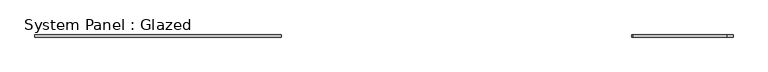
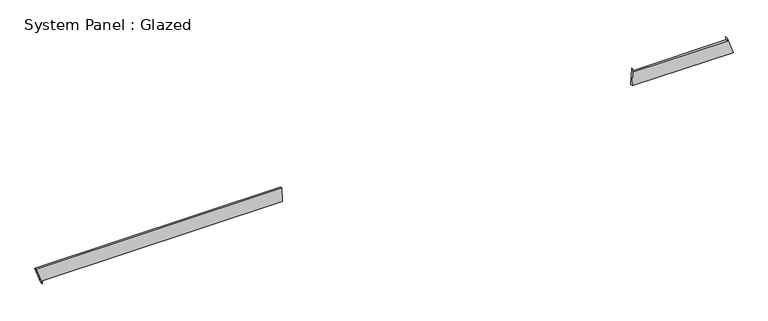
"""IFC4 building model written with IfcOpenShell, lengths in millimetres: plate geometry, System Panel : Glazed."""

from ifc_helpers import new_model, si_unit, frame, origin, place, context, project, spatial, polyline, outline, extrude, source, transform, mapped, element, save


def system_panel_glazed_9f0471fb(model_context):
    return source(origin(), model_context, "Body", "SweptSolid", [
        extrude(outline(polyline([(35.3553391, 2859.8495797), (35.3553391, 4027.1832678), (235.4605257, 3957.794267), (200.1051866, 3957.7948933), (200.0858758, 2867.7205954), (235.4412148, 2867.7199691), (35.3553391, 2859.8495797)])), frame((0.0, -49.5, 0.0), z_axis=(0.0, 1.0, 0.0), x_axis=(0.0, 0.0, 1.0)), (0.0, 0.0, 1.0), 25.0),
        extrude(outline(polyline([(0.0, -3957.4553629), (35.3553391, -3957.4553629), (35.3553391, -1184.8268191), (200.0140372, -1187.4748261), (199.9637313, -4027.1832678), (0.0, -3957.4553629)])), frame((0.0, -49.5, 0.0), z_axis=(0.0, 1.0, 0.0), x_axis=(0.0, 0.0, 1.0)), (0.0, 0.0, 1.0), 25.0),
    ])


if __name__ == "__main__":
    model = new_model("IFC4")
    model_context = context("Model", 3, world=origin())
    ifc_project = project(units=[si_unit("LENGTHUNIT", "METRE", prefix="MILLI")], contexts=[model_context])
    site = spatial("IfcSite", under=ifc_project)
    building = spatial("IfcBuilding", under=site)
    placement = place(None, origin())
    system_panel_glazed_shape = system_panel_glazed_9f0471fb(model_context)
    element("IfcPlate", 1, ObjectType="System Panel : Glazed", at=placement, inside=building, context=model_context, shape_type="MappedRepresentation", body=[
        mapped(system_panel_glazed_shape, transform((0.0, 0.0, 0.0), x_axis=(1.0, 0.0, 0.0), y_axis=(0.0, 1.0, 0.0), z_axis=(0.0, 0.0, 1.0))),
    ])
    save(model, "model.ifc")

# Revit data of these elements
# Element 1 (IfcPlate, "System Panel : Glazed")
#   Materials on its faces: "Glass"
# Materials
#   "Glass": class "Glass", colour RGB 218 227 224, transparency 0.85, Description = "Soda Lime Glass", Cost = 0
